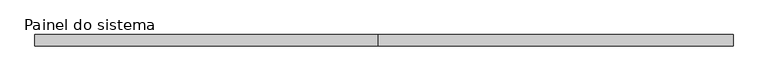
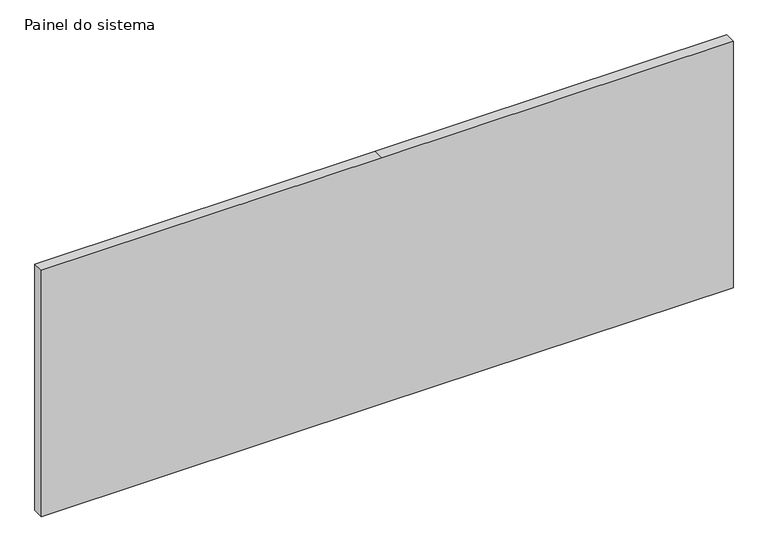
"""IFC4 building model written with IfcOpenShell, lengths in millimetres: plate geometry, Painel do sistema : Envidraçado."""

from ifc_helpers import new_model, si_unit, frame, origin, place, context, project, spatial, polyline, outline, extrude, source, transform, mapped, element, save


def painel_do_sistema_d52e1df4(model_context):
    return source(origin(), model_context, "Body", "SweptSolid", [
        extrude(outline(polyline([(0.0, -783.4833334), (0.0, -12.4999998), (0.0, 783.4833334), (590.0, 783.4833334), (590.0, -12.4999998), (590.0, -783.4833334), (0.0, -783.4833334)])), frame((0.0, -49.5, 0.0), z_axis=(0.0, 1.0, 0.0), x_axis=(0.0, 0.0, 1.0)), (0.0, 0.0, 1.0), 25.0),
    ])


if __name__ == "__main__":
    model = new_model("IFC4")
    model_context = context("Model", 3, world=origin())
    ifc_project = project(units=[si_unit("LENGTHUNIT", "METRE", prefix="MILLI")], contexts=[model_context])
    site = spatial("IfcSite", under=ifc_project)
    building = spatial("IfcBuilding", under=site)
    placement = place(None, origin())
    painel_do_sistema_shape = painel_do_sistema_d52e1df4(model_context)
    element("IfcPlate", 1, ObjectType="Painel do sistema : Envidraçado", at=placement, inside=building, context=model_context, shape_type="MappedRepresentation", body=[
        mapped(painel_do_sistema_shape, transform((0.0, 0.0, 0.0), x_axis=(1.0, 0.0, 0.0), y_axis=(0.0, 1.0, 0.0), z_axis=(0.0, 0.0, 1.0))),
    ])
    save(model, "model.ifc")

# Revit data of these elements
# Type "Painel do sistema : Envidraçado"
#   Construction Type Id = "GSP4R"
#   Analytic Construction = "Vidraça única Pilkington 1/8 pol"
#   Visual Light Transmittance = 0.9
#   Solar Heat Gain Coefficient = 0.86
#   Heat Transfer Coefficient (U) = 6.7069 W/(m²·K)
# Element 1 (IfcPlate, "Painel do sistema : Envidraçado")
#   Materials on its faces: ".VIDRO GENÉRICO"
# Materials
#   ".VIDRO GENÉRICO": class ".CC_VIDRO", colour RGB 0 128 192, transparency 0.9, Description = "Vidro comum", Cost = 0
